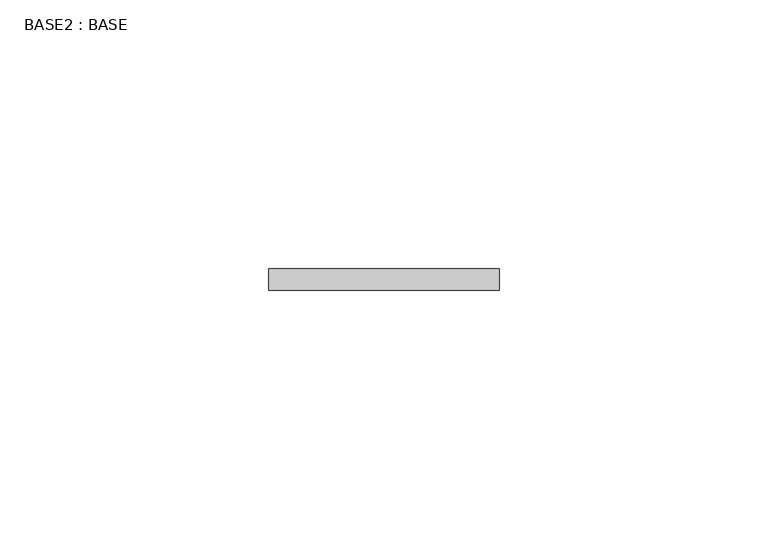
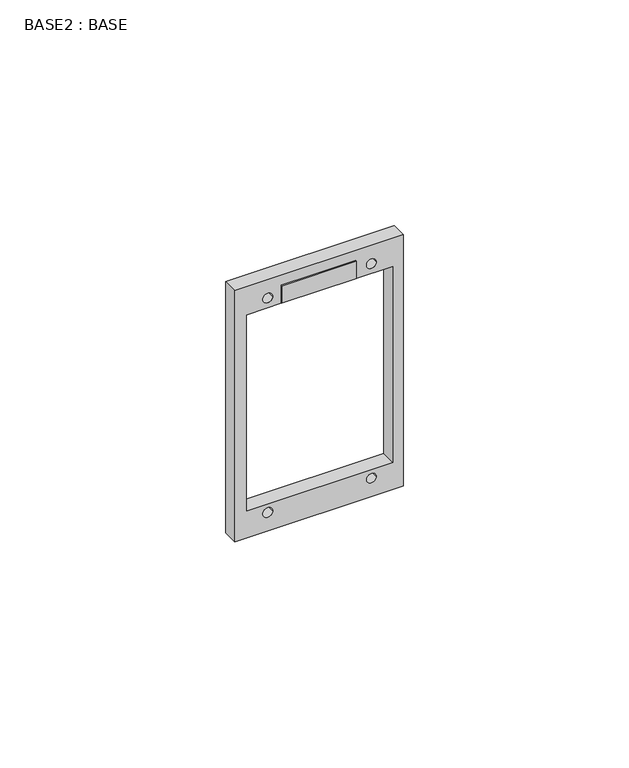
"""IFC4 building model written with IfcOpenShell, lengths in millimetres: proxy geometry, BASE2 : BASE."""

from ifc_helpers import new_model, si_unit, point, frame, frame_2d, origin, place, context, project, spatial, polyline, circle_curve, trimmed, segment, composite_curve, outline, extrude, source, transform, mapped, element, save


def base2_base_c05baaad(model_context):
    return source(origin(), model_context, "Body", "SweptSolid", [
        extrude(outline(polyline([(2465.0719295, 1293.4498458), (2465.0719295, 1291.7192449), (2446.0719295, 1291.7192449), (2446.0719295, 1293.4498458), (2465.0719295, 1293.4498458)])), frame((0.0, 0.0, 60.3), z_axis=(0.0, 0.0, 1.0), x_axis=(1.0, 0.0, 0.0)), (0.0, 0.0, 1.0), 4.7),
        extrude(outline(polyline([(0.0, 2434.0719295), (0.0, 2477.0719295), (68.0, 2477.0719295), (68.0, 2434.0719295), (0.0, 2434.0719295)]), holes=[composite_curve([segment(trimmed(circle_curve(frame_2d((63.0, 2468.9719295)), 1.25), [point((63.0, 2467.7219295))], [point((63.0, 2470.2219295))], True, "CARTESIAN"), True, "CONTINUOUS"), segment(trimmed(circle_curve(frame_2d((63.0, 2468.9719295)), 1.25), [point((63.0, 2470.2219295))], [point((63.0, 2467.7219295))], True, "CARTESIAN"), True, "CONTINUOUS")], self_intersect=False), composite_curve([segment(trimmed(circle_curve(frame_2d((5.0, 2468.9719295)), 1.25), [point((5.0, 2470.2219295))], [point((5.0, 2467.7219295))], True, "CARTESIAN"), True, "CONTINUOUS"), segment(trimmed(circle_curve(frame_2d((5.0, 2468.9719295)), 1.25), [point((5.0, 2467.7219295))], [point((5.0, 2470.2219295))], True, "CARTESIAN"), True, "CONTINUOUS")], self_intersect=False), composite_curve([segment(trimmed(circle_curve(frame_2d((5.0, 2442.4719295)), 1.25), [point((5.0, 2443.7219295))], [point((5.0, 2441.2219295))], True, "CARTESIAN"), True, "CONTINUOUS"), segment(trimmed(circle_curve(frame_2d((5.0, 2442.4719295)), 1.25), [point((5.0, 2441.2219295))], [point((5.0, 2443.7219295))], True, "CARTESIAN"), True, "CONTINUOUS")], self_intersect=False), composite_curve([segment(trimmed(circle_curve(frame_2d((63.0, 2442.4719295)), 1.25), [point((63.0, 2443.7219295))], [point((63.0, 2441.2219295))], True, "CARTESIAN"), True, "CONTINUOUS"), segment(trimmed(circle_curve(frame_2d((63.0, 2442.4719295)), 1.25), [point((63.0, 2441.2219295))], [point((63.0, 2443.7219295))], True, "CARTESIAN"), True, "CONTINUOUS")], self_intersect=False), polyline([(7.3, 2474.3719295), (7.3, 2437.0719295), (60.3, 2437.0719295), (60.3, 2446.0719295), (65.0, 2446.0719295), (65.0, 2465.0719295), (60.3, 2465.0719295), (60.3, 2474.3719295), (7.3, 2474.3719295)])]), frame((0.0, 1291.7192449, 0.0), z_axis=(0.0, 1.0, 0.0), x_axis=(0.0, 0.0, 1.0)), (0.0, 0.0, 1.0), 4.0),
    ])


if __name__ == "__main__":
    model = new_model("IFC4")
    model_context = context("Model", 3, world=origin())
    ifc_project = project(units=[si_unit("LENGTHUNIT", "METRE", prefix="MILLI")], contexts=[model_context])
    site = spatial("IfcSite", under=ifc_project)
    building = spatial("IfcBuilding", under=site)
    placement = place(None, origin())
    base2_base_shape = base2_base_c05baaad(model_context)
    element("IfcBuildingElementProxy", 1, Name="BASE2 : BASE", ObjectType="BASE2 : BASE", at=placement, inside=building, context=model_context, shape_type="MappedRepresentation", body=[
        mapped(base2_base_shape, transform((0.0, 0.0, 0.0), x_axis=(1.0, 0.0, 0.0), y_axis=(0.0, 1.0, 0.0), z_axis=(0.0, 0.0, 1.0))),
    ])
    save(model, "model.ifc")

# Revit data of these elements
# Element 1 (IfcBuildingElementProxy, "BASE2 : BASE")
#   Materials on its faces: ".BOX FUNDO"
# Materials
#   ".BOX FUNDO": class "Vidro", colour RGB 236 240 239, transparency 0.15, Cost = 0
